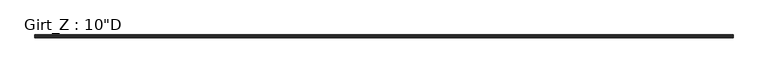
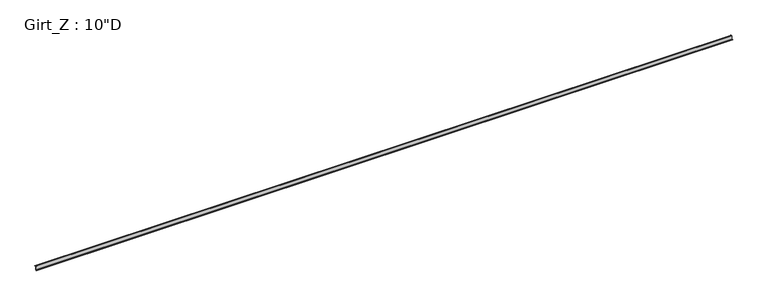
"""IFC4 building model written with IfcOpenShell, lengths in millimetres: beam geometry."""

from ifc_helpers import new_model, si_unit, point, frame, frame_2d, origin, place, context, project, spatial, polyline, circle_curve, trimmed, segment, composite_curve, outline, extrude, source, transform, mapped, element, save


def beam_96a2f50a(model_context):
    return source(origin(), model_context, "Body", "SweptSolid", [
        extrude(outline(composite_curve([segment(polyline([(77.9859375, 127.0), (90.2310415, 112.4068534), (88.1028742, 110.621109), (76.6904765, 124.221875), (3.3005807, 124.221875)]), True, "CONTINUOUS"), segment(trimmed(circle_curve(frame_2d((3.3741066, 122.2381931)), 1.9850441), [point((3.3005807, 124.221875))], [point((1.3890625, 122.2381931))], True, "CARTESIAN"), True, "CONTINUOUS"), segment(polyline([(1.3890625, 122.2381931), (1.3890625, -127.0), (-84.3359375, -127.0), (-96.5810415, -112.4068534), (-94.4528742, -110.621109), (-83.0404765, -124.221875), (-3.2694106, -124.221875)]), True, "CONTINUOUS"), segment(trimmed(circle_curve(frame_2d((-3.3748024, -122.2389339)), 1.9857399), [point((-3.2694106, -124.221875))], [point((-1.3890625, -122.2389339))], True, "CARTESIAN"), True, "CONTINUOUS"), segment(polyline([(-1.3890625, -122.2389339), (-1.3890625, 122.2375)]), True, "CONTINUOUS"), segment(trimmed(circle_curve(frame_2d((3.3734375, 122.2375)), 4.7625), [point((-1.3890625, 122.2375))], [point((3.3734375, 127.0))], False, "CARTESIAN"), True, "CONTINUOUS"), segment(polyline([(3.3734375, 127.0), (77.9859375, 127.0)]), True, "CONTINUOUS")], self_intersect=False)), frame((-24143.096875, 0.0, 0.0), z_axis=(1.0, 0.0, 0.0), x_axis=(0.0, 1.0, 0.0)), (0.0, 0.0, 1.0), 48120.3),
    ])


if __name__ == "__main__":
    model = new_model("IFC4")
    model_context = context("Model", 3, world=origin())
    ifc_project = project(units=[si_unit("LENGTHUNIT", "METRE", prefix="MILLI")], contexts=[model_context])
    site = spatial("IfcSite", under=ifc_project)
    building = spatial("IfcBuilding", under=site)
    placement = place(None, origin())
    beam_shape = beam_96a2f50a(model_context)
    element("IfcBeam", 1, ObjectType="Girt_Z : 10\"D", at=placement, inside=building, context=model_context, shape_type="MappedRepresentation", body=[
        mapped(beam_shape, transform((0.0, 0.0, 0.0), x_axis=(1.0, 0.0, 0.0), y_axis=(0.0, 1.0, 0.0), z_axis=(0.0, 0.0, 1.0))),
    ])
    save(model, "model.ifc")

# Revit data of these elements
# Type "Girt_Z : 10\"D"
#   half leg = 0' - 1 11/16"
#   Web_Thickness = 0' - 0 7/64"
#   Length [instance default] = 10' - 0"
#   Leg_2 = 0' - 3 3/8"
#   Leg_1 = 0' - 3 1/8"
#   Height = 0' - 10"
#   Structural Material [instance default] = none
# Element 1 (IfcBeam, "Girt_Z : 10\"D")
#   Structural Material = STRUCTURAL STEEL - SEE STRUCT. DWGS
#   Materials on its faces: "STRUCTURAL STEEL - SEE STRUCT. DWGS"
# Materials
#   "STRUCTURAL STEEL - SEE STRUCT. DWGS": class "Metal", colour RGB 137 146 153, transparency 0, Description = "Steel, mill finish", Cost = 0
